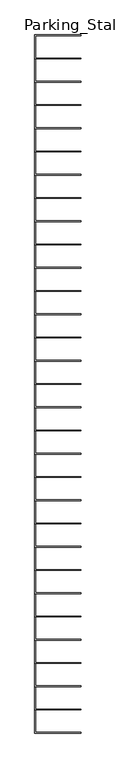
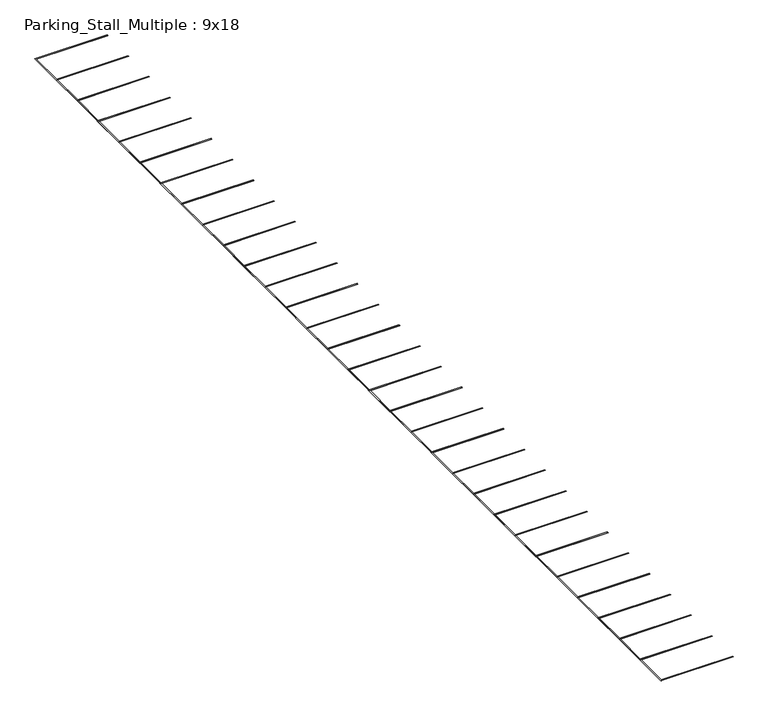
"""IFC4 building model written with IfcOpenShell, lengths in millimetres: proxy geometry, Parking_Stall_Multiple : 9x18."""

from ifc_helpers import new_model, si_unit, origin, origin_with_axes, place, context, project, spatial, polyline, outline, extrude, source, transform, mapped, element, save


def parking_stall_multiple_9x18_9dfe9d75(model_context):
    return source(origin(), model_context, "Body", "SweptSolid", [
        extrude(outline(polyline([(5486.4, 79552.8), (0.0, 79552.8), (0.0, 82372.2), (5486.4, 82372.2), (5486.4, 82296.0), (76.2, 82296.0), (76.2, 79629.0), (5486.4, 79629.0), (5486.4, 79552.8)])), origin_with_axes(), (0.0, 0.0, 1.0), 6.35),
        extrude(outline(polyline([(5486.4, 76809.6), (0.0, 76809.6), (0.0, 79629.0), (5486.4, 79629.0), (5486.4, 79552.8), (76.2, 79552.8), (76.2, 76885.8), (5486.4, 76885.8), (5486.4, 76809.6)])), origin_with_axes(), (0.0, 0.0, 1.0), 6.35),
        extrude(outline(polyline([(5486.4, 74066.4), (0.0, 74066.4), (0.0, 76885.8), (5486.4, 76885.8), (5486.4, 76809.6), (76.2, 76809.6), (76.2, 74142.6), (5486.4, 74142.6), (5486.4, 74066.4)])), origin_with_axes(), (0.0, 0.0, 1.0), 6.35),
        extrude(outline(polyline([(5486.4, 71323.2), (0.0, 71323.2), (0.0, 74142.6), (5486.4, 74142.6), (5486.4, 74066.4), (76.2, 74066.4), (76.2, 71399.4), (5486.4, 71399.4), (5486.4, 71323.2)])), origin_with_axes(), (0.0, 0.0, 1.0), 6.35),
        extrude(outline(polyline([(5486.4, 68580.0), (0.0, 68580.0), (0.0, 71399.4), (5486.4, 71399.4), (5486.4, 71323.2), (76.2, 71323.2), (76.2, 68656.2), (5486.4, 68656.2), (5486.4, 68580.0)])), origin_with_axes(), (0.0, 0.0, 1.0), 6.35),
        extrude(outline(polyline([(5486.4, 65836.8), (0.0, 65836.8), (0.0, 68656.2), (5486.4, 68656.2), (5486.4, 68580.0), (76.2, 68580.0), (76.2, 65913.0), (5486.4, 65913.0), (5486.4, 65836.8)])), origin_with_axes(), (0.0, 0.0, 1.0), 6.35),
        extrude(outline(polyline([(5486.4, 63093.6), (0.0, 63093.6), (0.0, 65913.0), (5486.4, 65913.0), (5486.4, 65836.8), (76.2, 65836.8), (76.2, 63169.8), (5486.4, 63169.8), (5486.4, 63093.6)])), origin_with_axes(), (0.0, 0.0, 1.0), 6.35),
        extrude(outline(polyline([(5486.4, 60350.4), (0.0, 60350.4), (0.0, 63169.8), (5486.4, 63169.8), (5486.4, 63093.6), (76.2, 63093.6), (76.2, 60426.6), (5486.4, 60426.6), (5486.4, 60350.4)])), origin_with_axes(), (0.0, 0.0, 1.0), 6.35),
        extrude(outline(polyline([(5486.4, 57607.2), (0.0, 57607.2), (0.0, 60426.6), (5486.4, 60426.6), (5486.4, 60350.4), (76.2, 60350.4), (76.2, 57683.4), (5486.4, 57683.4), (5486.4, 57607.2)])), origin_with_axes(), (0.0, 0.0, 1.0), 6.35),
        extrude(outline(polyline([(5486.4, 54864.0), (0.0, 54864.0), (0.0, 57683.4), (5486.4, 57683.4), (5486.4, 57607.2), (76.2, 57607.2), (76.2, 54940.2), (5486.4, 54940.2), (5486.4, 54864.0)])), origin_with_axes(), (0.0, 0.0, 1.0), 6.35),
        extrude(outline(polyline([(5486.4, 52120.8), (0.0, 52120.8), (0.0, 54940.2), (5486.4, 54940.2), (5486.4, 54864.0), (76.2, 54864.0), (76.2, 52197.0), (5486.4, 52197.0), (5486.4, 52120.8)])), origin_with_axes(), (0.0, 0.0, 1.0), 6.35),
        extrude(outline(polyline([(5486.4, 49377.6), (0.0, 49377.6), (0.0, 52197.0), (5486.4, 52197.0), (5486.4, 52120.8), (76.2, 52120.8), (76.2, 49453.8), (5486.4, 49453.8), (5486.4, 49377.6)])), origin_with_axes(), (0.0, 0.0, 1.0), 6.35),
        extrude(outline(polyline([(5486.4, 46634.4), (0.0, 46634.4), (0.0, 49453.8), (5486.4, 49453.8), (5486.4, 49377.6), (76.2, 49377.6), (76.2, 46710.6), (5486.4, 46710.6), (5486.4, 46634.4)])), origin_with_axes(), (0.0, 0.0, 1.0), 6.35),
        extrude(outline(polyline([(5486.4, 43891.2), (0.0, 43891.2), (0.0, 46710.6), (5486.4, 46710.6), (5486.4, 46634.4), (76.2, 46634.4), (76.2, 43967.4), (5486.4, 43967.4), (5486.4, 43891.2)])), origin_with_axes(), (0.0, 0.0, 1.0), 6.35),
        extrude(outline(polyline([(5486.4, 41148.0), (0.0, 41148.0), (0.0, 43967.4), (5486.4, 43967.4), (5486.4, 43891.2), (76.2, 43891.2), (76.2, 41224.2), (5486.4, 41224.2), (5486.4, 41148.0)])), origin_with_axes(), (0.0, 0.0, 1.0), 6.35),
        extrude(outline(polyline([(5486.4, 38404.8), (0.0, 38404.8), (0.0, 41224.2), (5486.4, 41224.2), (5486.4, 41148.0), (76.2, 41148.0), (76.2, 38481.0), (5486.4, 38481.0), (5486.4, 38404.8)])), origin_with_axes(), (0.0, 0.0, 1.0), 6.35),
        extrude(outline(polyline([(5486.4, 35661.6), (0.0, 35661.6), (0.0, 38481.0), (5486.4, 38481.0), (5486.4, 38404.8), (76.2, 38404.8), (76.2, 35737.8), (5486.4, 35737.8), (5486.4, 35661.6)])), origin_with_axes(), (0.0, 0.0, 1.0), 6.35),
        extrude(outline(polyline([(5486.4, 32918.4), (0.0, 32918.4), (0.0, 35737.8), (5486.4, 35737.8), (5486.4, 35661.6), (76.2, 35661.6), (76.2, 32994.6), (5486.4, 32994.6), (5486.4, 32918.4)])), origin_with_axes(), (0.0, 0.0, 1.0), 6.35),
        extrude(outline(polyline([(5486.4, 30175.2), (0.0, 30175.2), (0.0, 32994.6), (5486.4, 32994.6), (5486.4, 32918.4), (76.2, 32918.4), (76.2, 30251.4), (5486.4, 30251.4), (5486.4, 30175.2)])), origin_with_axes(), (0.0, 0.0, 1.0), 6.35),
        extrude(outline(polyline([(5486.4, 27432.0), (0.0, 27432.0), (0.0, 30251.4), (5486.4, 30251.4), (5486.4, 30175.2), (76.2, 30175.2), (76.2, 27508.2), (5486.4, 27508.2), (5486.4, 27432.0)])), origin_with_axes(), (0.0, 0.0, 1.0), 6.35),
        extrude(outline(polyline([(5486.4, 24688.8), (0.0, 24688.8), (0.0, 27508.2), (5486.4, 27508.2), (5486.4, 27432.0), (76.2, 27432.0), (76.2, 24765.0), (5486.4, 24765.0), (5486.4, 24688.8)])), origin_with_axes(), (0.0, 0.0, 1.0), 6.35),
        extrude(outline(polyline([(5486.4, 21945.6), (0.0, 21945.6), (0.0, 24765.0), (5486.4, 24765.0), (5486.4, 24688.8), (76.2, 24688.8), (76.2, 22021.8), (5486.4, 22021.8), (5486.4, 21945.6)])), origin_with_axes(), (0.0, 0.0, 1.0), 6.35),
        extrude(outline(polyline([(5486.4, 19202.4), (0.0, 19202.4), (0.0, 22021.8), (5486.4, 22021.8), (5486.4, 21945.6), (76.2, 21945.6), (76.2, 19278.6), (5486.4, 19278.6), (5486.4, 19202.4)])), origin_with_axes(), (0.0, 0.0, 1.0), 6.35),
        extrude(outline(polyline([(5486.4, 16459.2), (0.0, 16459.2), (0.0, 19278.6), (5486.4, 19278.6), (5486.4, 19202.4), (76.2, 19202.4), (76.2, 16535.4), (5486.4, 16535.4), (5486.4, 16459.2)])), origin_with_axes(), (0.0, 0.0, 1.0), 6.35),
        extrude(outline(polyline([(5486.4, 13716.0), (0.0, 13716.0), (0.0, 16535.4), (5486.4, 16535.4), (5486.4, 16459.2), (76.2, 16459.2), (76.2, 13792.2), (5486.4, 13792.2), (5486.4, 13716.0)])), origin_with_axes(), (0.0, 0.0, 1.0), 6.35),
        extrude(outline(polyline([(5486.4, 10972.8), (0.0, 10972.8), (0.0, 13792.2), (5486.4, 13792.2), (5486.4, 13716.0), (76.2, 13716.0), (76.2, 11049.0), (5486.4, 11049.0), (5486.4, 10972.8)])), origin_with_axes(), (0.0, 0.0, 1.0), 6.35),
        extrude(outline(polyline([(5486.4, 8229.6), (0.0, 8229.6), (0.0, 11049.0), (5486.4, 11049.0), (5486.4, 10972.8), (76.2, 10972.8), (76.2, 8305.8), (5486.4, 8305.8), (5486.4, 8229.6)])), origin_with_axes(), (0.0, 0.0, 1.0), 6.35),
        extrude(outline(polyline([(5486.4, 5486.4), (0.0, 5486.4), (0.0, 8305.8), (5486.4, 8305.8), (5486.4, 8229.6), (76.2, 8229.6), (76.2, 5562.6), (5486.4, 5562.6), (5486.4, 5486.4)])), origin_with_axes(), (0.0, 0.0, 1.0), 6.35),
        extrude(outline(polyline([(5486.4, 2743.2), (0.0, 2743.2), (0.0, 5562.6), (5486.4, 5562.6), (5486.4, 5486.4), (76.2, 5486.4), (76.2, 2819.4), (5486.4, 2819.4), (5486.4, 2743.2)])), origin_with_axes(), (0.0, 0.0, 1.0), 6.35),
        extrude(outline(polyline([(5486.4, 0.0), (0.0, 0.0), (0.0, 2819.4), (5486.4, 2819.4), (5486.4, 2743.2), (76.2, 2743.2), (76.2, 76.2), (5486.4, 76.2), (5486.4, 0.0)])), origin_with_axes(), (0.0, 0.0, 1.0), 6.35),
    ])


if __name__ == "__main__":
    model = new_model("IFC4")
    model_context = context("Model", 3, world=origin())
    ifc_project = project(units=[si_unit("LENGTHUNIT", "METRE", prefix="MILLI")], contexts=[model_context])
    site = spatial("IfcSite", under=ifc_project)
    building = spatial("IfcBuilding", under=site)
    placement = place(None, origin())
    parking_stall_multiple_9x18_shape = parking_stall_multiple_9x18_9dfe9d75(model_context)
    element("IfcBuildingElementProxy", 1, Name="Parking_Stall_Multiple : 9x18", ObjectType="Parking_Stall_Multiple : 9x18", at=placement, inside=building, context=model_context, shape_type="MappedRepresentation", body=[
        mapped(parking_stall_multiple_9x18_shape, transform((0.0, 0.0, 0.0), x_axis=(1.0, 0.0, 0.0), y_axis=(0.0, 1.0, 0.0), z_axis=(0.0, 0.0, 1.0))),
    ])
    save(model, "model.ifc")

# Revit data of these elements
# Type "Parking_Stall_Multiple : 9x18"
#   Type Mark = "PK-1"
#   Parking_Width_M = 9' - 0"
#   Parking_Run_Length [instance default] = 65' - 0"
#   Parking_Line_Width = 0' - 3"
#   Parking_Length_M = 18' - 0"
#   Single_Parking_Visibility [instance default] = no
#   Parking_ADA_Symbol = no
#   ParkingUnitsArray [instance default] = 7
#   ParkingUnits [instance default] = 7
#   Multiple_Parking_Visibility [instance default] = yes
#   Parking_Line_Material = none
# Element 1 (IfcBuildingElementProxy, "Parking_Stall_Multiple : 9x18")
#   Parking_Run_Length = 266' - 3.19592"
#   ParkingUnitsArray = 30
#   ParkingUnits = 30
